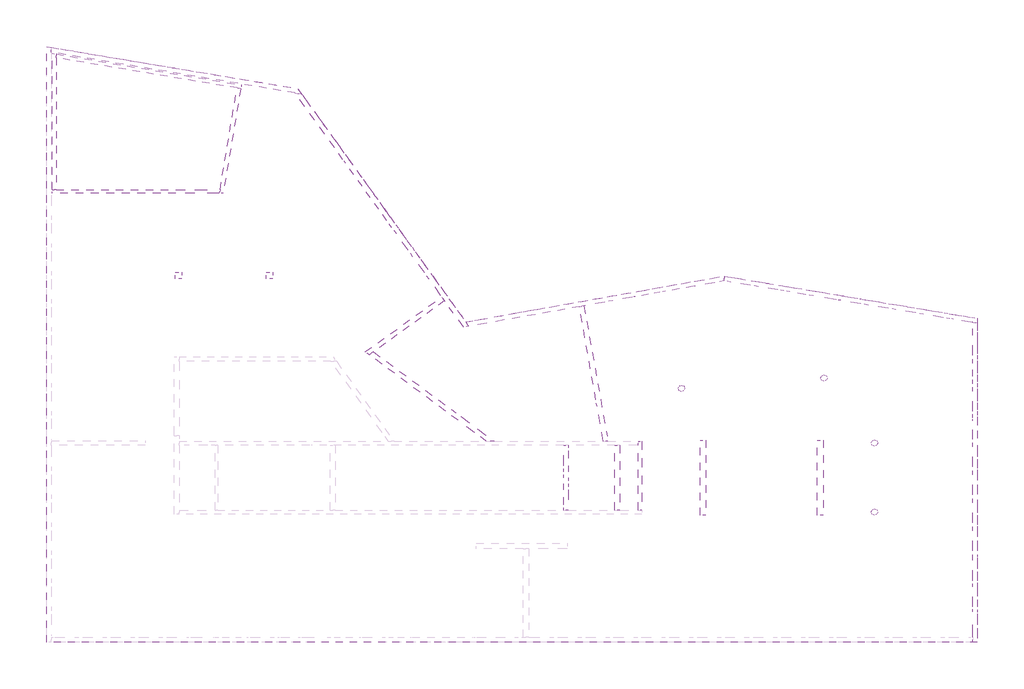
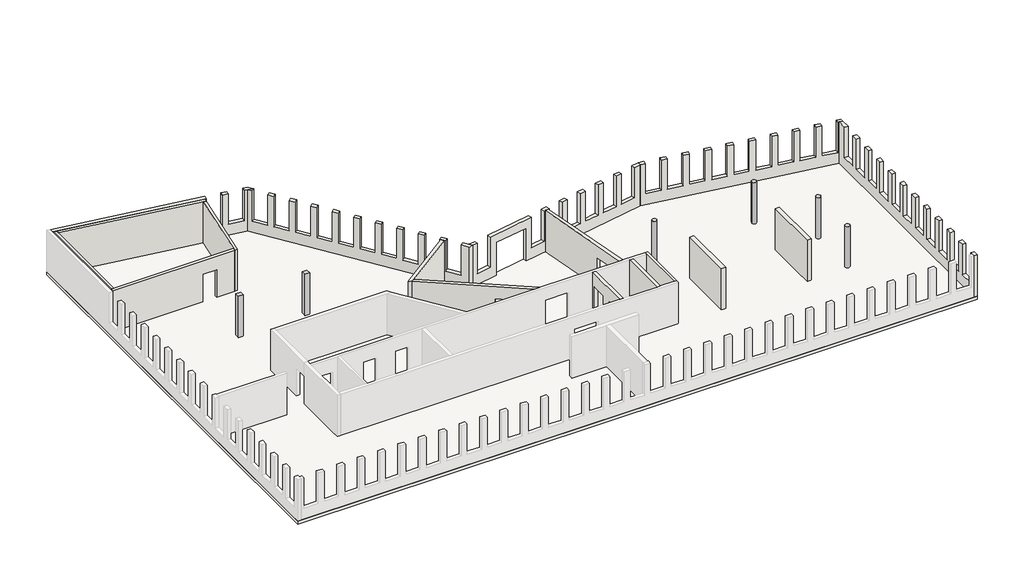
# One storey, part 2 of 2: 17 walls, 6 columns, 1 slab.
"""IFC4 building model written with IfcOpenShell, lengths in millimetres."""

from ifc_helpers import new_model, si_unit, point, frame, frame_2d, origin, place, context, project, spatial, polyline, circle_curve, trimmed, segment, composite_curve, outline, extrude, faceted_brep, element, save

model = new_model("IFC4")

# Units and contexts
model_context = context("Model", 3, world=origin())
ifc_project = project(units=[si_unit("LENGTHUNIT", "METRE", prefix="MILLI")], contexts=[model_context])

# Site, building, storey
site = spatial("IfcSite", under=ifc_project)
building = spatial("IfcBuilding", under=site)
storey = spatial("IfcBuildingStorey", under=building, Name="01_UG_OKFB_-4,20", Elevation=-4200.0)

# Columns
placement = place(None, origin())
element("IfcColumn", 1, ObjectType="5dki STB-Stützen rund : 5dki Stütze rund ø35cm C40/50", at=placement, inside=storey, context=model_context, shape_type="SweptSolid", body=[
    extrude(outline(composite_curve([segment(trimmed(circle_curve(frame_2d((33961.7583834, 13503.0230367)), 175.0), [point((34136.7583834, 13503.0230367))], [point((33786.7583834, 13503.0230367))], False, "CARTESIAN"), True, "CONTINUOUS"), segment(trimmed(circle_curve(frame_2d((33961.7583834, 13503.0230367)), 175.0), [point((33786.7583834, 13503.0230367))], [point((34136.7583834, 13503.0230367))], False, "CARTESIAN"), True, "CONTINUOUS")], self_intersect=False)), frame((0.0, 0.0, -150.0), z_axis=(0.0, 0.0, 1.0), x_axis=(1.0, 0.0, 0.0)), (0.0, 0.0, 1.0), 3210.0),
])
element("IfcColumn", 2, ObjectType="5dki STB-Stützen rechteckig : 5dki Stütze recht. 35x35cm C35/45", at=placement, inside=storey, context=model_context, shape_type="SweptSolid", body=[
    extrude(outline(polyline([(7139.9999521, 19742.0124565), (7139.9999521, 19392.0124565), (6789.9999521, 19392.0124565), (6789.9999521, 19742.0124565), (7139.9999521, 19742.0124565)])), frame((0.0, 0.0, -150.0), z_axis=(0.0, 0.0, 1.0), x_axis=(1.0, 0.0, 0.0)), (0.0, 0.0, 1.0), 3210.0),
])
element("IfcColumn", 3, ObjectType="5dki STB-Stützen rechteckig : 5dki Stütze recht. 35x35cm C35/45", at=placement, inside=storey, context=model_context, shape_type="SweptSolid", body=[
    extrude(outline(polyline([(12021.4450432, 19742.0124565), (12021.4450432, 19392.0124565), (11671.4450432, 19392.0124565), (11671.4450432, 19742.0124565), (12021.4450432, 19742.0124565)])), frame((0.0, 0.0, -150.0), z_axis=(0.0, 0.0, 1.0), x_axis=(1.0, 0.0, 0.0)), (0.0, 0.0, 1.0), 3210.0),
])
element("IfcColumn", 4, ObjectType="5dki STB-Stützen rund : 5dki Stütze rund ø35cm C40/50", at=placement, inside=storey, context=model_context, shape_type="SweptSolid", body=[
    extrude(outline(composite_curve([segment(trimmed(circle_curve(frame_2d((41616.0718251, 14052.9332427)), 175.0), [point((41791.0718251, 14052.9332427))], [point((41441.0718251, 14052.9332427))], False, "CARTESIAN"), True, "CONTINUOUS"), segment(trimmed(circle_curve(frame_2d((41616.0718251, 14052.9332427)), 175.0), [point((41441.0718251, 14052.9332427))], [point((41791.0718251, 14052.9332427))], False, "CARTESIAN"), True, "CONTINUOUS")], self_intersect=False)), frame((0.0, 0.0, -150.0), z_axis=(0.0, 0.0, 1.0), x_axis=(1.0, 0.0, 0.0)), (0.0, 0.0, 1.0), 3210.0),
])
element("IfcColumn", 5, ObjectType="5dki STB-Stützen rund : 5dki Stütze rund ø35cm C40/50", at=placement, inside=storey, context=model_context, shape_type="SweptSolid", body=[
    extrude(outline(composite_curve([segment(trimmed(circle_curve(frame_2d((44328.9990923, 10566.8309986)), 175.0), [point((44503.9990923, 10566.8309986))], [point((44153.9990923, 10566.8309986))], False, "CARTESIAN"), True, "CONTINUOUS"), segment(trimmed(circle_curve(frame_2d((44328.9990923, 10566.8309986)), 175.0), [point((44153.9990923, 10566.8309986))], [point((44503.9990923, 10566.8309986))], False, "CARTESIAN"), True, "CONTINUOUS")], self_intersect=False)), frame((0.0, 0.0, -150.0), z_axis=(0.0, 0.0, 1.0), x_axis=(1.0, 0.0, 0.0)), (0.0, 0.0, 1.0), 3210.0),
])
element("IfcColumn", 6, ObjectType="5dki STB-Stützen rund : 5dki Stütze rund ø35cm C40/50", at=placement, inside=storey, context=model_context, shape_type="SweptSolid", body=[
    extrude(outline(composite_curve([segment(trimmed(circle_curve(frame_2d((44328.9990923, 6852.1619165)), 175.0), [point((44503.9990923, 6852.1619165))], [point((44153.9990923, 6852.1619165))], False, "CARTESIAN"), True, "CONTINUOUS"), segment(trimmed(circle_curve(frame_2d((44328.9990923, 6852.1619165)), 175.0), [point((44153.9990923, 6852.1619165))], [point((44503.9990923, 6852.1619165))], False, "CARTESIAN"), True, "CONTINUOUS")], self_intersect=False)), frame((0.0, 0.0, -150.0), z_axis=(0.0, 0.0, 1.0), x_axis=(1.0, 0.0, 0.0)), (0.0, 0.0, 1.0), 3210.0),
])

# Slab
element("IfcSlab", 7, ObjectType="5dki Decke Ortbeton 25cm C30/37", at=placement, inside=storey, context=model_context, shape_type="SweptSolid", body=[
    extrude(outline(polyline([(13359.8955456, 29603.0548931), (22383.504194, 17069.412817), (36259.255712, 19532.4198889), (49863.9990834, 17260.5812626), (49863.9990834, -129.9989509), (-129.9989953, -129.9989509), (-129.9989953, 31855.7150729), (13359.8955456, 29603.0548931)]), holes=[polyline([(30391.9999833, 10442.0127412), (27891.9999829, 10442.0127412), (27891.9999829, 6960.0000515), (30391.9999833, 6960.0000515), (30391.9999833, 10442.0127412)]), polyline([(31652.9293554, 10442.0127466), (30641.9999891, 10442.0127466), (30641.9999891, 6948.5225137), (31652.9293554, 6948.5225137), (31652.9293554, 10442.0127466)]), polyline([(8916.9999838, 10442.0127045), (6990.0003593, 10442.0127045), (6990.0003593, 6960.0000208), (8916.9999838, 6960.0000208), (8916.9999838, 10442.0127045)]), polyline([(24127.0004657, 8820.0328918), (16927.0004692, 8820.0328918), (16927.0004692, 7020.033352), (24127.0004657, 7020.033352), (24127.0004657, 8820.0328918)])]), frame((0.0, 0.0, -400.0), z_axis=(0.0, 0.0, 1.0), x_axis=(1.0, 0.0, 0.0)), (0.0, 0.0, 1.0), 250.0),
])

# Walls
element("IfcWall", 8, ObjectType="5dki Lochfassade 26cm C30/37", at=placement, inside=storey, context=model_context, shape_type="Brep", body=[
    faceted_brep([(13575.6085618, 29303.4331075, 3060.0), (13211.4553837, 29364.2425792, 3060.0), (12991.7792945, 29400.9260074, 3060.0), (12991.7792945, 29400.9260074, 710.0), (11926.5295409, 29578.8106961, 710.0), (11926.5295409, 29578.8106961, 3060.0), (11512.2657479, 29647.9880751, 3060.0), (11512.2657479, 29647.9880751, 710.0), (10447.0159943, 29825.8727639, 710.0), (10447.0159943, 29825.8727639, 3060.0), (130.0010047, 31548.6978518, 3060.0), (130.0010047, 31548.6978518, -150.0), (13211.4553837, 29364.2425792, -150.0), (13575.6085618, 29303.4331075, -150.0), (13034.6033862, 29657.3750221, 710.0), (13034.6033862, 29657.3750221, 3060.0), (13359.8955383, 29603.0549033, 3060.0), (13359.8955383, 29603.0549033, -150.0), (130.0010047, 31812.2980067, -150.0), (130.0010047, 31812.2980067, 3060.0), (10489.840086, 30082.3217786, 3060.0), (10489.840086, 30082.3217786, 710.0), (11555.0898396, 29904.4370898, 710.0), (11555.0898396, 29904.4370898, 3060.0), (11969.3536327, 29835.2597109, 3060.0), (11969.3536327, 29835.2597109, 710.0)], [[[0, 1, 2, 3, 4, 5, 6, 7, 8, 9, 10, 11, 12, 13]], [[14, 15, 16, 17, 18, 19, 20, 21, 22, 23, 24, 25]], [[13, 12, 11, 18, 17]], [[19, 10, 9, 20]], [[24, 23, 6, 5]], [[16, 15, 2, 1, 0]], [[11, 10, 19, 18]], [[0, 13, 17, 16]], [[8, 21, 20, 9]], [[22, 7, 6, 23]], [[21, 8, 7, 22]], [[5, 4, 25, 24]], [[3, 2, 15, 14]], [[4, 3, 14, 25]]]),
])
element("IfcWall", 9, ObjectType="5dki Lochfassade 26cm C30/37", at=placement, inside=storey, context=model_context, shape_type="Brep", body=[
    faceted_brep([(22268.004401, 16784.8468851, 3060.0), (21924.4906268, 17261.9817942, 3060.0), (21924.4906268, 17261.9817942, 710.0), (21293.4697845, 18138.4592307, 710.0), (21293.4697845, 18138.4592307, 3060.0), (21048.0727903, 18479.3115671, 3060.0), (21048.0727903, 18479.3115671, 710.0), (20417.0519481, 19355.7890035, 710.0), (20417.0519481, 19355.7890035, 3060.0), (20171.6549538, 19696.64134, 3060.0), (20171.6549538, 19696.64134, 710.0), (19540.6341116, 20573.1187764, 710.0), (19540.6341116, 20573.1187764, 3060.0), (19295.2371174, 20913.9711128, 3060.0), (19295.2371174, 20913.9711128, 710.0), (18664.2162751, 21790.4485493, 710.0), (18664.2162751, 21790.4485493, 3060.0), (18418.8192809, 22131.3008857, 3060.0), (18418.8192809, 22131.3008857, 710.0), (17787.7984387, 23007.7783222, 710.0), (17787.7984387, 23007.7783222, 3060.0), (17542.4014445, 23348.6306586, 3060.0), (17542.4014445, 23348.6306586, 710.0), (16911.3806022, 24225.1080951, 710.0), (16911.3806022, 24225.1080951, 3060.0), (16665.983608, 24565.9604315, 3060.0), (16665.983608, 24565.9604315, 710.0), (16034.9627658, 25442.4378679, 710.0), (16034.9627658, 25442.4378679, 3060.0), (15789.5657715, 25783.2902043, 3060.0), (15789.5657715, 25783.2902043, 710.0), (15158.5449293, 26659.7676408, 710.0), (15158.5449293, 26659.7676408, 3060.0), (14913.1479351, 27000.6199772, 3060.0), (14913.1479351, 27000.6199772, 710.0), (14282.1270928, 27877.0974137, 710.0), (14282.1270928, 27877.0974137, 3060.0), (14036.7300986, 28217.9497501, 3060.0), (14036.7300986, 28217.9497501, 710.0), (13405.7092564, 29094.4271866, 710.0), (13405.7092564, 29094.4271866, 3060.0), (13211.4553837, 29364.2425792, 3060.0), (13211.4553837, 29364.2425792, -150.0), (22268.004401, 16784.8468851, -150.0), (22135.4944541, 17413.8942192, 710.0), (22135.4944541, 17413.8942192, 3060.0), (22383.5041721, 17069.4128529, 3060.0), (22552.0750732, 16835.2706799, 3060.0), (22552.0750732, 16835.2706799, -150.0), (22383.5041721, 17069.4128529, -150.0), (13575.6085618, 29303.4331075, -150.0), (13575.6085618, 29303.4331075, 3060.0), (13616.7130837, 29246.3396115, 3060.0), (13616.7130837, 29246.3396115, 710.0), (14247.7339259, 28369.8621751, 710.0), (14247.7339259, 28369.8621751, 3060.0), (14493.1309201, 28029.0098387, 3060.0), (14493.1309201, 28029.0098387, 710.0), (15124.1517624, 27152.5324022, 710.0), (15124.1517624, 27152.5324022, 3060.0), (15369.5487566, 26811.6800658, 3060.0), (15369.5487566, 26811.6800658, 710.0), (16000.5695988, 25935.2026293, 710.0), (16000.5695988, 25935.2026293, 3060.0), (16245.966593, 25594.3502929, 3060.0), (16245.966593, 25594.3502929, 710.0), (16876.9874353, 24717.8728564, 710.0), (16876.9874353, 24717.8728564, 3060.0), (17122.3844295, 24377.02052, 3060.0), (17122.3844295, 24377.02052, 710.0), (17753.4052718, 23500.5430836, 710.0), (17753.4052718, 23500.5430836, 3060.0), (17998.802266, 23159.6907472, 3060.0), (17998.802266, 23159.6907472, 710.0), (18629.8231082, 22283.2133107, 710.0), (18629.8231082, 22283.2133107, 3060.0), (18875.2201024, 21942.3609743, 3060.0), (18875.2201024, 21942.3609743, 710.0), (19506.2409447, 21065.8835378, 710.0), (19506.2409447, 21065.8835378, 3060.0), (19751.6379389, 20725.0312014, 3060.0), (19751.6379389, 20725.0312014, 710.0), (20382.6587811, 19848.5537649, 710.0), (20382.6587811, 19848.5537649, 3060.0), (20628.0557754, 19507.7014285, 3060.0), (20628.0557754, 19507.7014285, 710.0), (21259.0766176, 18631.2239921, 710.0), (21259.0766176, 18631.2239921, 3060.0), (21504.4736118, 18290.3716557, 3060.0), (21504.4736118, 18290.3716557, 710.0)], [[[0, 1, 2, 3, 4, 5, 6, 7, 8, 9, 10, 11, 12, 13, 14, 15, 16, 17, 18, 19, 20, 21, 22, 23, 24, 25, 26, 27, 28, 29, 30, 31, 32, 33, 34, 35, 36, 37, 38, 39, 40, 41, 42, 43]], [[44, 45, 46, 47, 48, 49, 50, 51, 52, 53, 54, 55, 56, 57, 58, 59, 60, 61, 62, 63, 64, 65, 66, 67, 68, 69, 70, 71, 72, 73, 74, 75, 76, 77, 78, 79, 80, 81, 82, 83, 84, 85, 86, 87, 88, 89]], [[43, 42, 50, 49, 48]], [[51, 41, 40, 52]], [[56, 55, 37, 36]], [[60, 59, 33, 32]], [[64, 63, 29, 28]], [[68, 67, 25, 24]], [[72, 71, 21, 20]], [[76, 75, 17, 16]], [[80, 79, 13, 12]], [[84, 83, 9, 8]], [[88, 87, 5, 4]], [[47, 46, 45, 1, 0]], [[42, 41, 51, 50]], [[0, 43, 48, 47]], [[39, 53, 52, 40]], [[54, 38, 37, 55]], [[53, 39, 38, 54]], [[36, 35, 57, 56]], [[34, 33, 59, 58]], [[35, 34, 58, 57]], [[32, 31, 61, 60]], [[30, 29, 63, 62]], [[31, 30, 62, 61]], [[28, 27, 65, 64]], [[26, 25, 67, 66]], [[27, 26, 66, 65]], [[24, 23, 69, 68]], [[22, 21, 71, 70]], [[23, 22, 70, 69]], [[20, 19, 73, 72]], [[18, 17, 75, 74]], [[19, 18, 74, 73]], [[16, 15, 77, 76]], [[14, 13, 79, 78]], [[15, 14, 78, 77]], [[12, 11, 81, 80]], [[10, 9, 83, 82]], [[11, 10, 82, 81]], [[8, 7, 85, 84]], [[6, 5, 87, 86]], [[7, 6, 86, 85]], [[4, 3, 89, 88]], [[2, 1, 45, 44]], [[3, 2, 44, 89]]]),
])
element("IfcWall", 10, ObjectType="5dki Lochfassade 26cm C30/37", at=placement, inside=storey, context=model_context, shape_type="Brep", body=[
    faceted_brep([(34703.2430153, 18992.1564787, 710.0), (34703.2430153, 18992.1564787, 3060.0), (34289.7072944, 18918.7520679, 3060.0), (34289.7072944, 18918.7520679, 710.0), (33226.3297263, 18729.9978686, 710.0), (33226.3297263, 18729.9978686, 3060.0), (32812.7940054, 18656.5934577, 3060.0), (32812.7940054, 18656.5934577, 710.0), (31749.4164374, 18467.8392585, 710.0), (31749.4164374, 18467.8392585, 3060.0), (31335.8807164, 18394.4348476, 3060.0), (31335.8807164, 18394.4348476, 710.0), (30272.5031484, 18205.6806483, 710.0), (30272.5031484, 18205.6806483, 3060.0), (29858.9674275, 18132.2762375, 3060.0), (29858.9674275, 18132.2762375, 710.0), (28795.5898594, 17943.5220382, 710.0), (28795.5898594, 17943.5220382, 3060.0), (28731.5904499, 17932.1618613, 3060.0), (28485.4382351, 17888.4687596, 3060.0), (28382.0541385, 17870.1176274, 3060.0), (28382.0541385, 17870.1176274, 710.0), (27318.6765704, 17681.3634281, 710.0), (27318.6765704, 17681.3634281, 3060.0), (23971.0064488, 17087.1372452, 3060.0), (23971.0064488, 17087.1372452, 710.0), (22907.6288807, 16898.3830459, 710.0), (22907.6288807, 16898.3830459, 3060.0), (22552.0750732, 16835.2706799, 3060.0), (22552.0750732, 16835.2706799, -150.0), (24463.3121553, 17174.5236752, -150.0), (24463.3121553, 17174.5236752, 2410.0), (26924.8343036, 17611.454692, 2410.0), (26924.8343036, 17611.454692, -150.0), (28485.4382351, 17888.4687596, -150.0), (28731.5904499, 17932.1618613, -150.0), (36261.33607, 19268.7248546, -150.0), (36261.33607, 19268.7248546, 3060.0), (35766.6205834, 19180.910678, 3060.0), (35766.6205834, 19180.910678, 710.0), (34244.2664686, 19174.7503713, 3060.0), (34657.8021895, 19248.1547821, 3060.0), (34657.8021895, 19248.1547821, 710.0), (35721.1797576, 19436.9089814, 710.0), (35721.1797576, 19436.9089814, 3060.0), (36259.9888873, 19532.5499737, 3060.0), (36259.9888873, 19532.5499737, -150.0), (26879.3934778, 17867.4529955, -150.0), (26879.3934778, 17867.4529955, 2410.0), (24417.8713295, 17430.5219786, 2410.0), (24417.8713295, 17430.5219786, -150.0), (22383.5041721, 17069.4128529, -150.0), (22383.5041721, 17069.4128529, 3060.0), (22862.188055, 17154.3813493, 3060.0), (22862.188055, 17154.3813493, 710.0), (23925.565623, 17343.1355486, 710.0), (23925.565623, 17343.1355486, 3060.0), (27273.2357447, 17937.3617315, 3060.0), (27273.2357447, 17937.3617315, 710.0), (28336.6133127, 18126.1159308, 710.0), (28336.6133127, 18126.1159308, 3060.0), (28750.1490337, 18199.5203416, 3060.0), (28750.1490337, 18199.5203416, 710.0), (29813.5266017, 18388.2745409, 710.0), (29813.5266017, 18388.2745409, 3060.0), (30227.0623226, 18461.6789518, 3060.0), (30227.0623226, 18461.6789518, 710.0), (31290.4398907, 18650.433151, 710.0), (31290.4398907, 18650.433151, 3060.0), (31703.9756116, 18723.8375619, 3060.0), (31703.9756116, 18723.8375619, 710.0), (32767.3531797, 18912.5917612, 710.0), (32767.3531797, 18912.5917612, 3060.0), (33180.8889006, 18985.996172, 3060.0), (33180.8889006, 18985.996172, 710.0), (34244.2664686, 19174.7503713, 710.0)], [[[0, 1, 2, 3, 4, 5, 6, 7, 8, 9, 10, 11, 12, 13, 14, 15, 16, 17, 18, 19, 20, 21, 22, 23, 24, 25, 26, 27, 28, 29, 30, 31, 32, 33, 34, 35, 36, 37, 38, 39]], [[40, 41, 42, 43, 44, 45, 46, 47, 48, 49, 50, 51, 52, 53, 54, 55, 56, 57, 58, 59, 60, 61, 62, 63, 64, 65, 66, 67, 68, 69, 70, 71, 72, 73, 74, 75]], [[29, 51, 50, 30]], [[46, 36, 35, 34, 33, 47]], [[53, 52, 28, 27]], [[24, 23, 57, 56]], [[61, 60, 20, 19, 18, 17]], [[14, 13, 65, 64]], [[69, 68, 10, 9]], [[6, 5, 73, 72]], [[38, 37, 45, 44]], [[2, 1, 41, 40]], [[29, 28, 52, 51]], [[37, 36, 46, 45]], [[49, 31, 30, 50]], [[31, 49, 48, 32]], [[32, 48, 47, 33]], [[27, 26, 54, 53]], [[25, 24, 56, 55]], [[26, 25, 55, 54]], [[60, 59, 21, 20]], [[58, 57, 23, 22]], [[59, 58, 22, 21]], [[17, 16, 62, 61]], [[15, 14, 64, 63]], [[16, 15, 63, 62]], [[68, 67, 11, 10]], [[66, 65, 13, 12]], [[67, 66, 12, 11]], [[9, 8, 70, 69]], [[7, 6, 72, 71]], [[8, 7, 71, 70]], [[40, 75, 3, 2]], [[74, 73, 5, 4]], [[75, 74, 4, 3]], [[44, 43, 39, 38]], [[42, 41, 1, 0]], [[43, 42, 0, 39]]]),
])
element("IfcWall", 11, ObjectType="5dki Lochfassade 26cm C30/37", at=placement, inside=storey, context=model_context, shape_type="Brep", body=[
    faceted_brep([(49863.9990837, 16997.2336245, 3060.0), (49603.9990837, 17040.6506907, 3060.0), (49507.8677901, 17056.7035319, 3060.0), (49507.8677901, 17056.7035319, 710.0), (48442.6180365, 17234.5882205, 710.0), (48442.6180365, 17234.5882205, 3060.0), (48028.3542434, 17303.7655993, 3060.0), (48028.3542434, 17303.7655993, 710.0), (46963.1044898, 17481.6502878, 710.0), (46963.1044898, 17481.6502878, 3060.0), (46548.8406967, 17550.8276667, 3060.0), (46548.8406967, 17550.8276667, 710.0), (45483.5909431, 17728.7123552, 710.0), (45483.5909431, 17728.7123552, 3060.0), (45069.32715, 17797.8897341, 3060.0), (45069.32715, 17797.8897341, 710.0), (44004.0773964, 17975.7744226, 710.0), (44004.0773964, 17975.7744226, 3060.0), (43589.8136033, 18044.9518015, 3060.0), (43589.8136033, 18044.9518015, 710.0), (42524.5638497, 18222.83649, 710.0), (42524.5638497, 18222.83649, 3060.0), (42110.3000566, 18292.0138689, 3060.0), (42110.3000566, 18292.0138689, 710.0), (41045.050303, 18469.8985574, 710.0), (41045.050303, 18469.8985574, 3060.0), (40630.7865099, 18539.0759362, 3060.0), (40630.7865099, 18539.0759362, 710.0), (39565.5367563, 18716.9606248, 710.0), (39565.5367563, 18716.9606248, 3060.0), (39151.2729632, 18786.1380036, 3060.0), (39151.2729632, 18786.1380036, 710.0), (38086.0232096, 18964.0226921, 710.0), (38086.0232096, 18964.0226921, 3060.0), (37671.7594165, 19033.200071, 3060.0), (37671.7594165, 19033.200071, 710.0), (36606.5096629, 19211.0847595, 710.0), (36606.5096629, 19211.0847595, 3060.0), (36261.33607, 19268.7248546, 3060.0), (36261.33607, 19268.7248546, -150.0), (49603.9990837, 17040.6506907, -150.0), (49863.9990837, 16997.2336245, -150.0), (49550.6918818, 17313.1525467, 710.0), (49550.6918818, 17313.1525467, 3060.0), (49863.9990833, 17260.8337794, 3060.0), (49863.9990833, 17260.8337794, -150.0), (36259.9888873, 19532.5499737, -150.0), (36259.9888873, 19532.5499737, 3060.0), (36649.3337546, 19467.5337743, 3060.0), (36649.3337546, 19467.5337743, 710.0), (37714.5835082, 19289.6490858, 710.0), (37714.5835082, 19289.6490858, 3060.0), (38128.8473013, 19220.4717069, 3060.0), (38128.8473013, 19220.4717069, 710.0), (39194.0970549, 19042.5870184, 710.0), (39194.0970549, 19042.5870184, 3060.0), (39608.360848, 18973.4096395, 3060.0), (39608.360848, 18973.4096395, 710.0), (40673.6106016, 18795.524951, 710.0), (40673.6106016, 18795.524951, 3060.0), (41087.8743947, 18726.3475721, 3060.0), (41087.8743947, 18726.3475721, 710.0), (42153.1241483, 18548.4628836, 710.0), (42153.1241483, 18548.4628836, 3060.0), (42567.3879414, 18479.2855048, 3060.0), (42567.3879414, 18479.2855048, 710.0), (43632.637695, 18301.4008162, 710.0), (43632.637695, 18301.4008162, 3060.0), (44046.9014881, 18232.2234374, 3060.0), (44046.9014881, 18232.2234374, 710.0), (45112.1512417, 18054.3387489, 710.0), (45112.1512417, 18054.3387489, 3060.0), (45526.4150348, 17985.16137, 3060.0), (45526.4150348, 17985.16137, 710.0), (46591.6647884, 17807.2766815, 710.0), (46591.6647884, 17807.2766815, 3060.0), (47005.9285815, 17738.0993026, 3060.0), (47005.9285815, 17738.0993026, 710.0), (48071.1783351, 17560.2146141, 710.0), (48071.1783351, 17560.2146141, 3060.0), (48485.4421282, 17491.0372352, 3060.0), (48485.4421282, 17491.0372352, 710.0)], [[[0, 1, 2, 3, 4, 5, 6, 7, 8, 9, 10, 11, 12, 13, 14, 15, 16, 17, 18, 19, 20, 21, 22, 23, 24, 25, 26, 27, 28, 29, 30, 31, 32, 33, 34, 35, 36, 37, 38, 39, 40, 41]], [[42, 43, 44, 45, 46, 47, 48, 49, 50, 51, 52, 53, 54, 55, 56, 57, 58, 59, 60, 61, 62, 63, 64, 65, 66, 67, 68, 69, 70, 71, 72, 73, 74, 75, 76, 77, 78, 79, 80, 81]], [[41, 40, 39, 46, 45]], [[48, 47, 38, 37]], [[52, 51, 34, 33]], [[56, 55, 30, 29]], [[60, 59, 26, 25]], [[64, 63, 22, 21]], [[68, 67, 18, 17]], [[72, 71, 14, 13]], [[76, 75, 10, 9]], [[80, 79, 6, 5]], [[44, 43, 2, 1, 0]], [[39, 38, 47, 46]], [[0, 41, 45, 44]], [[37, 36, 49, 48]], [[35, 34, 51, 50]], [[36, 35, 50, 49]], [[33, 32, 53, 52]], [[31, 30, 55, 54]], [[32, 31, 54, 53]], [[29, 28, 57, 56]], [[27, 26, 59, 58]], [[28, 27, 58, 57]], [[25, 24, 61, 60]], [[23, 22, 63, 62]], [[24, 23, 62, 61]], [[21, 20, 65, 64]], [[19, 18, 67, 66]], [[20, 19, 66, 65]], [[17, 16, 69, 68]], [[15, 14, 71, 70]], [[16, 15, 70, 69]], [[13, 12, 73, 72]], [[11, 10, 75, 74]], [[12, 11, 74, 73]], [[9, 8, 77, 76]], [[7, 6, 79, 78]], [[8, 7, 78, 77]], [[5, 4, 81, 80]], [[3, 2, 43, 42]], [[4, 3, 42, 81]]]),
])
element("IfcWall", 12, ObjectType="5dki Lochfassade 26cm C30/37", at=placement, inside=storey, context=model_context, shape_type="Brep", body=[
    faceted_brep([(49603.9991105, -129.9989514, 3060.0), (49603.9991101, 130.0010486, 3060.0), (49603.9991099, 277.0124979, 3060.0), (49603.9991099, 277.0124979, 710.0), (49603.9991082, 1357.0124979, 710.0), (49603.9991082, 1357.0124979, 3060.0), (49603.9991075, 1777.0124979, 3060.0), (49603.9991075, 1777.0124979, 710.0), (49603.9991058, 2857.0124979, 710.0), (49603.9991058, 2857.0124979, 3060.0), (49603.9991052, 3277.0124979, 3060.0), (49603.9991052, 3277.0124979, 710.0), (49603.9991035, 4357.0124979, 710.0), (49603.9991035, 4357.0124979, 3060.0), (49603.9991028, 4777.0124979, 3060.0), (49603.9991028, 4777.0124979, 710.0), (49603.9991011, 5857.0124979, 710.0), (49603.9991011, 5857.0124979, 3060.0), (49603.9991005, 6277.0124979, 3060.0), (49603.9991005, 6277.0124979, 710.0), (49603.9990988, 7357.0124979, 710.0), (49603.9990988, 7357.0124979, 3060.0), (49603.9990981, 7777.0124979, 3060.0), (49603.9990981, 7777.0124979, 710.0), (49603.9990964, 8857.0124979, 710.0), (49603.9990964, 8857.0124979, 3060.0), (49603.9990958, 9277.0124979, 3060.0), (49603.9990958, 9277.0124979, 710.0), (49603.9990941, 10357.0124979, 710.0), (49603.9990941, 10357.0124979, 3060.0), (49603.9990934, 10777.0124979, 3060.0), (49603.9990934, 10777.0124979, 710.0), (49603.9990918, 11857.0124979, 710.0), (49603.9990918, 11857.0124979, 3060.0), (49603.9990911, 12277.0124979, 3060.0), (49603.9990911, 12277.0124979, 710.0), (49603.9990894, 13357.0124979, 710.0), (49603.9990894, 13357.0124979, 3060.0), (49603.9990888, 13777.0124979, 3060.0), (49603.9990888, 13777.0124979, 710.0), (49603.9990871, 14857.0124979, 710.0), (49603.9990871, 14857.0124979, 3060.0), (49603.9990864, 15277.0124979, 3060.0), (49603.9990864, 15277.0124979, 710.0), (49603.9990847, 16357.0124979, 710.0), (49603.9990847, 16357.0124979, 3060.0), (49603.9990837, 17040.6506907, 3060.0), (49603.9990837, 17040.6506907, -150.0), (49603.9991101, 130.0010486, -150.0), (49603.9991105, -129.9989514, -150.0), (49863.9991099, 277.0124983, 710.0), (49863.9991099, 277.0124983, 3060.0), (49863.9991105, -129.9989509, 3060.0), (49863.9991105, -129.9989509, -150.0), (49863.9990837, 16997.2336245, -150.0), (49863.9990837, 16997.2336245, 3060.0), (49863.9990847, 16357.0124983, 3060.0), (49863.9990847, 16357.0124983, 710.0), (49863.9990864, 15277.0124983, 710.0), (49863.9990864, 15277.0124983, 3060.0), (49863.9990871, 14857.0124983, 3060.0), (49863.9990871, 14857.0124983, 710.0), (49863.9990888, 13777.0124983, 710.0), (49863.9990888, 13777.0124983, 3060.0), (49863.9990894, 13357.0124983, 3060.0), (49863.9990894, 13357.0124983, 710.0), (49863.9990911, 12277.0124983, 710.0), (49863.9990911, 12277.0124983, 3060.0), (49863.9990918, 11857.0124983, 3060.0), (49863.9990918, 11857.0124983, 710.0), (49863.9990934, 10777.0124983, 710.0), (49863.9990934, 10777.0124983, 3060.0), (49863.9990941, 10357.0124983, 3060.0), (49863.9990941, 10357.0124983, 710.0), (49863.9990958, 9277.0124983, 710.0), (49863.9990958, 9277.0124983, 3060.0), (49863.9990964, 8857.0124983, 3060.0), (49863.9990964, 8857.0124983, 710.0), (49863.9990981, 7777.0124983, 710.0), (49863.9990981, 7777.0124983, 3060.0), (49863.9990988, 7357.0124983, 3060.0), (49863.9990988, 7357.0124983, 710.0), (49863.9991005, 6277.0124983, 710.0), (49863.9991005, 6277.0124983, 3060.0), (49863.9991011, 5857.0124983, 3060.0), (49863.9991011, 5857.0124983, 710.0), (49863.9991028, 4777.0124983, 710.0), (49863.9991028, 4777.0124983, 3060.0), (49863.9991035, 4357.0124983, 3060.0), (49863.9991035, 4357.0124983, 710.0), (49863.9991052, 3277.0124983, 710.0), (49863.9991052, 3277.0124983, 3060.0), (49863.9991058, 2857.0124983, 3060.0), (49863.9991058, 2857.0124983, 710.0), (49863.9991075, 1777.0124983, 710.0), (49863.9991075, 1777.0124983, 3060.0), (49863.9991082, 1357.0124983, 3060.0), (49863.9991082, 1357.0124983, 710.0)], [[[0, 1, 2, 3, 4, 5, 6, 7, 8, 9, 10, 11, 12, 13, 14, 15, 16, 17, 18, 19, 20, 21, 22, 23, 24, 25, 26, 27, 28, 29, 30, 31, 32, 33, 34, 35, 36, 37, 38, 39, 40, 41, 42, 43, 44, 45, 46, 47, 48, 49]], [[50, 51, 52, 53, 54, 55, 56, 57, 58, 59, 60, 61, 62, 63, 64, 65, 66, 67, 68, 69, 70, 71, 72, 73, 74, 75, 76, 77, 78, 79, 80, 81, 82, 83, 84, 85, 86, 87, 88, 89, 90, 91, 92, 93, 94, 95, 96, 97]], [[49, 48, 47, 54, 53]], [[55, 46, 45, 56]], [[42, 41, 60, 59]], [[38, 37, 64, 63]], [[34, 33, 68, 67]], [[30, 29, 72, 71]], [[26, 25, 76, 75]], [[22, 21, 80, 79]], [[18, 17, 84, 83]], [[14, 13, 88, 87]], [[10, 9, 92, 91]], [[96, 95, 6, 5]], [[52, 51, 2, 1, 0]], [[47, 46, 55, 54]], [[0, 49, 53, 52]], [[58, 43, 42, 59]], [[44, 57, 56, 45]], [[43, 58, 57, 44]], [[63, 62, 39, 38]], [[61, 60, 41, 40]], [[62, 61, 40, 39]], [[67, 66, 35, 34]], [[65, 64, 37, 36]], [[66, 65, 36, 35]], [[71, 70, 31, 30]], [[69, 68, 33, 32]], [[70, 69, 32, 31]], [[75, 74, 27, 26]], [[73, 72, 29, 28]], [[74, 73, 28, 27]], [[79, 78, 23, 22]], [[77, 76, 25, 24]], [[78, 77, 24, 23]], [[83, 82, 19, 18]], [[81, 80, 21, 20]], [[82, 81, 20, 19]], [[87, 86, 15, 14]], [[85, 84, 17, 16]], [[86, 85, 16, 15]], [[91, 90, 11, 10]], [[89, 88, 13, 12]], [[90, 89, 12, 11]], [[95, 94, 7, 6]], [[93, 92, 9, 8]], [[94, 93, 8, 7]], [[5, 4, 97, 96]], [[3, 2, 51, 50]], [[4, 3, 50, 97]]]),
])
element("IfcWall", 13, ObjectType="5dki STB-Wand Kern 25cm C30/37", at=placement, inside=storey, context=model_context, shape_type="SweptSolid", body=[
    extrude(outline(polyline([(30641.9999891, 10442.0127483), (30641.9999891, 6960.0000501), (30391.9999891, 6960.0000498), (30391.9999891, 10442.0127479), (30641.9999891, 10442.0127483)])), frame((0.0, 0.0, -150.0), z_axis=(0.0, 0.0, 1.0), x_axis=(1.0, 0.0, 0.0)), (0.0, 0.0, 1.0), 3210.0),
])
element("IfcWall", 14, ObjectType="5dki STB-Wand Kern 25cm C30/37", at=placement, inside=storey, context=model_context, shape_type="SweptSolid", body=[
    extrude(outline(polyline([(3482.0126944, -3210.0), (-2.1e-06, -3210.0), (-2.1e-06, 0.0), (279.9681323, 0.0), (279.9681323, -2260.0), (1414.9681323, -2260.0), (1414.9681323, 0.0), (2067.1995869, 0.0), (2067.1995869, -2260.0), (3202.1995869, -2260.0), (3202.1995869, 0.0), (3482.0126944, 0.0), (3482.0126944, -3210.0)])), frame((27641.9999829, 10442.0127408, -150.0), z_axis=(1.0, 1.6300916066412081e-09, 0.0), x_axis=(1.6300916066412081e-09, -1.0, 0.0)), (0.0, 0.0, 1.0), 250.0),
])
element("IfcWall", 15, ObjectType="5dki STB-Wand Kern 20cm C35/45", at=placement, inside=storey, context=model_context, shape_type="Brep", body=[
    faceted_brep([(31641.9999912, 10662.0127502, -150.0), (31641.9999881, 10442.0127502, -150.0), (31641.9999382, 6960.0000514, -150.0), (31641.9999382, 6960.0000514, 3060.0), (31641.9999881, 10442.0127502, 3060.0), (31641.9999912, 10662.0127502, 3060.0), (31841.9999912, 10662.0127505, -150.0), (31841.9999912, 10662.0127505, 3060.0), (31841.9999382, 6960.0000516, 3060.0), (31841.9999382, 6960.0000516, -150.0)], [[[0, 1, 2, 3, 4, 5]], [[6, 7, 8, 9]], [[2, 1, 0, 6, 9]], [[5, 4, 3, 8, 7]], [[0, 5, 7, 6]], [[3, 2, 9, 8]]]),
])
element("IfcWall", 16, ObjectType="5dki STB-Wand 20cm C30/37", at=placement, inside=storey, context=model_context, shape_type="Brep", body=[
    faceted_brep([(179.9999842, 24166.8495132, 3060.0), (379.9999842, 24166.8495132, 3060.0), (9187.7304791, 24166.8495132, 3060.0), (9187.7304791, 24166.8495132, -150.0), (7830.000204, 24166.8495132, -150.0), (7830.000204, 24166.8495132, 1985.0), (6820.000204, 24166.8495132, 1985.0), (6820.000204, 24166.8495132, -150.0), (379.9999842, 24166.8495132, -150.0), (179.9999842, 24166.8495132, -150.0), (9154.332736, 23966.8495132, 3060.0), (179.9999842, 23966.8495132, 3060.0), (179.9999842, 23966.8495132, -150.0), (6820.000204, 23966.8495132, -150.0), (6820.000204, 23966.8495132, 1985.0), (7830.000204, 23966.8495132, 1985.0), (7830.000204, 23966.8495132, -150.0), (9154.332736, 23966.8495132, -150.0)], [[[0, 1, 2, 3, 4, 5, 6, 7, 8, 9]], [[10, 11, 12, 13, 14, 15, 16, 17]], [[12, 9, 8, 7, 13]], [[3, 17, 16, 4]], [[2, 1, 0, 11, 10]], [[0, 9, 12, 11]], [[3, 2, 10, 17]], [[15, 5, 4, 16]], [[5, 15, 14, 6]], [[6, 14, 13, 7]]]),
])
element("IfcWall", 17, ObjectType="5dki STB-Wand 20cm C30/37", at=placement, inside=storey, context=model_context, shape_type="Brep", body=[
    faceted_brep([(379.9999842, 24166.8495132, -150.0), (379.9999842, 31253.489127, -150.0), (379.9999842, 31456.2584769, -150.0), (379.9999842, 31456.2584769, 3060.0), (379.9999842, 31253.489127, 3060.0), (379.9999842, 24166.8495132, 3060.0), (179.9999842, 24166.8495132, -150.0), (179.9999842, 24166.8495132, 3060.0), (179.9999842, 31489.6562201, 3060.0), (179.9999842, 31489.6562201, -150.0)], [[[0, 1, 2, 3, 4, 5]], [[6, 7, 8, 9]], [[2, 1, 0, 6, 9]], [[5, 4, 3, 8, 7]], [[0, 5, 7, 6]], [[3, 2, 9, 8]]]),
])
element("IfcWall", 18, ObjectType="5dki STB-Wand 20cm C30/37", at=placement, inside=storey, context=model_context, shape_type="Brep", body=[
    faceted_brep([(379.9999842, 31253.489127, -150.0), (10100.0728462, 29630.3466386, -150.0), (10297.3413191, 29597.4050296, -150.0), (10297.3413191, 29597.4050296, 3060.0), (10100.0728462, 29630.3466386, 3060.0), (379.9999842, 31253.489127, 3060.0), (379.9999842, 31456.2584769, -150.0), (379.9999842, 31456.2584769, 3060.0), (10330.282928, 29794.6735025, 3060.0), (10330.282928, 29794.6735025, -150.0)], [[[0, 1, 2, 3, 4, 5]], [[6, 7, 8, 9]], [[2, 1, 0, 6, 9]], [[5, 4, 3, 8, 7]], [[0, 5, 7, 6]], [[3, 2, 9, 8]]]),
])
element("IfcWall", 19, ObjectType="5dki STB-Wand 20cm C30/37", at=placement, inside=storey, context=model_context, shape_type="Brep", body=[
    faceted_brep([(10100.0728462, 29630.3466386, -150.0), (9187.7304791, 24166.8495132, -150.0), (9154.332736, 23966.8495132, -150.0), (9154.332736, 23966.8495132, 3060.0), (9187.7304791, 24166.8495132, 3060.0), (10100.0728462, 29630.3466386, 3060.0), (10297.3413191, 29597.4050296, -150.0), (10297.3413191, 29597.4050296, 3060.0), (9357.1020859, 23966.8495132, 3060.0), (9357.1020859, 23966.8495132, -150.0)], [[[0, 1, 2, 3, 4, 5]], [[6, 7, 8, 9]], [[2, 1, 0, 6, 9]], [[5, 4, 3, 8, 7]], [[0, 5, 7, 6]], [[3, 2, 9, 8]]]),
])
element("IfcWall", 20, ObjectType="5dki STB-Wand 25cm C30/37", at=placement, inside=storey, context=model_context, shape_type="Brep", body=[
    faceted_brep([(21084.845921, 18397.4352698, -150.0), (16996.4717259, 15463.7807738, -150.0), (16996.4717259, 15463.7807738, 3060.0), (21084.845921, 18397.4352698, 3060.0), (21230.5955347, 18194.3169542, -150.0), (21230.5955347, 18194.3169542, 3060.0), (17421.0951098, 15460.7711691, 3060.0), (17207.6873918, 15307.63829, 3060.0), (17207.6873918, 15307.63829, -150.0), (17421.0951098, 15460.7711691, -150.0)], [[[0, 1, 2, 3]], [[4, 5, 6, 7, 8, 9]], [[1, 0, 4, 9, 8]], [[3, 2, 7, 6, 5]], [[0, 3, 5, 4]], [[2, 1, 8, 7]]]),
])
element("IfcWall", 21, ObjectType="5dki STB-Wand 25cm C30/37", at=placement, inside=storey, context=model_context, shape_type="Brep", body=[
    faceted_brep([(23491.8764947, 10662.0127353, 3060.0), (17207.6873918, 15307.63829, 3060.0), (17207.6873918, 15307.63829, -150.0), (21455.778452, 12167.2107719, -150.0), (21455.778452, 12167.2107719, 2110.0), (22871.0433991, 11120.9674304, 2110.0), (22871.0433991, 11120.9674304, -150.0), (23491.8764947, 10662.0127353, -150.0), (17421.0951098, 15460.7711691, 3060.0), (23912.428752, 10662.0127361, 3060.0), (23912.428752, 10662.0127361, -150.0), (23019.6575101, 11321.9993832, -150.0), (23019.6575101, 11321.9993832, 2110.0), (21604.392563, 12368.2427246, 2110.0), (21604.392563, 12368.2427246, -150.0), (17421.0951098, 15460.7711691, -150.0)], [[[0, 1, 2, 3, 4, 5, 6, 7]], [[8, 9, 10, 11, 12, 13, 14, 15]], [[2, 15, 14, 3]], [[10, 7, 6, 11]], [[1, 0, 9, 8]], [[2, 1, 8, 15]], [[0, 7, 10, 9]], [[5, 12, 11, 6]], [[12, 5, 4, 13]], [[13, 4, 3, 14]]]),
])
element("IfcWall", 22, ObjectType="5dki STB-Wand 25cm C30/37", at=placement, inside=storey, context=model_context, shape_type="Brep", body=[
    faceted_brep([(29768.165987, 10662.0127467, 3060.0), (28485.4382351, 17888.4687596, 3060.0), (28485.4382351, 17888.4687596, -150.0), (29375.0297859, 12876.809659, -150.0), (29375.0297859, 12876.809659, 2110.0), (29682.6292216, 11143.8980666, 2110.0), (29682.6292216, 11143.8980666, -150.0), (29768.165987, 10662.0127467, -150.0), (28731.5904499, 17932.1618613, 3060.0), (30022.0739196, 10662.0127472, 3060.0), (30022.0739196, 10662.0127472, -150.0), (29928.7814364, 11187.5911682, -150.0), (29928.7814364, 11187.5911682, 2110.0), (29621.1820008, 12920.5027606, 2110.0), (29621.1820008, 12920.5027606, -150.0), (28731.5904499, 17932.1618613, -150.0)], [[[0, 1, 2, 3, 4, 5, 6, 7]], [[8, 9, 10, 11, 12, 13, 14, 15]], [[2, 15, 14, 3]], [[10, 7, 6, 11]], [[1, 0, 9, 8]], [[2, 1, 8, 15]], [[0, 7, 10, 9]], [[5, 12, 11, 6]], [[12, 5, 4, 13]], [[13, 4, 3, 14]]]),
])
element("IfcWall", 23, ObjectType="5dki STB-Wand 30cm C30/37", at=placement, inside=storey, context=model_context, shape_type="SweptSolid", body=[
    extrude(outline(polyline([(34969.9990839, 6680.0000532), (34969.9990776, 10702.0125181), (35269.9990776, 10702.0125186), (35269.9990839, 6680.0000537), (34969.9990839, 6680.0000532)])), frame((0.0, 0.0, -150.0), z_axis=(0.0, 0.0, 1.0), x_axis=(1.0, 0.0, 0.0)), (0.0, 0.0, 1.0), 3210.0),
])
element("IfcWall", 24, ObjectType="5dki STB-Wand 30cm C30/37", at=placement, inside=storey, context=model_context, shape_type="SweptSolid", body=[
    extrude(outline(polyline([(41269.9990703, 6680.000074), (41269.9990703, 10722.0122605), (41569.9990703, 10722.0122605), (41569.9990703, 6680.000074), (41269.9990703, 6680.000074)])), frame((0.0, 0.0, -150.0), z_axis=(0.0, 0.0, 1.0), x_axis=(1.0, 0.0, 0.0)), (0.0, 0.0, 1.0), 3210.0),
])

save(model, "model.ifc")

# Revit data of these elements
# Type "5dki STB-Stützen rund : 5dki Stütze rund ø35cm C40/50"
#   cpiFitMatchKey = "5D-KI-STB-OB-ST-RUN"
#   cpiComponentType = "Column"
#   5d Materialgüte = "C40/50"
#   Radius = 0.175 m
#   Durchmesser = 0.350 m
#   5dki Bewehrung Stab kg pro m3 = 0
#   5dki Sichtbeton SB3/SB4 [instance default] = no
#   Structural Material = 5d Beton - Stahlbeton
#   Assembly Code = ""
# Type "5dki STB-Stützen rechteckig : 5dki Stütze recht. 35x35cm C35/45"
#   cpiFitMatchKey = "5D-KI-STB-OB-ST-REC"
#   cpiComponentType = "Column"
#   5d Materialgüte = "C35/45"
#   Tiefe = 0.350 m
#   Breite = 0.350 m
#   5dki Bewehrung Stab kg pro m3 = 0
#   5dki Sichtbeton SB3/SB4 [instance default] = no
#   Structural Material = 5d Beton - Stahlbeton
#   Assembly Code = ""
# Type "5dki Decke Ortbeton 25cm C30/37"
#   cpiComponentType = "Slab"
#   cpiFitMatchKey = "5D-KI-STB-OB-DE"
#   5d Materialgüte = "C30/37"
#   Function = 0
#   5dki WU = no
#   Layers, outside or top first: 0.250 m "5d Beton - Stahlbeton" (function 1)
# Type "5dki Lochfassade 26cm C30/37"
#   Type Comments = ""
#   Description = ""
#   cpiComponentType = "Wall"
#   cpiFitMatchKey = "5D-KI-STB-OB-W-LF"
#   5d Materialgüte = "C35/45"
#   Filter Tragend / Nichttragend = yes
#   5dki WU = no
#   Layers, outside or top first: 0.260 m "5d Beton - Stahlbeton" (function 1)
# Type "5dki STB-Wand Kern 25cm C30/37"
#   Type Comments = ""
#   Description = ""
#   cpiComponentType = "Wall"
#   cpiFitMatchKey = "5D-KI-STB-OB-W-K"
#   5d Materialgüte = "C30/37"
#   Filter Tragend / Nichttragend = yes
#   5dki WU = no
#   Layers, outside or top first: 0.250 m "5d Beton - Stahlbeton" (function 1)
# Type "5dki STB-Wand Kern 20cm C35/45"
#   Type Comments = ""
#   Description = ""
#   cpiComponentType = "Wall"
#   cpiFitMatchKey = "5D-KI-STB-OB-W-K"
#   5d Materialgüte = "C35/45"
#   Filter Tragend / Nichttragend = yes
#   5dki WU = no
#   Layers, outside or top first: 0.200 m "5d Beton - Stahlbeton" (function 1)
# Type "5dki STB-Wand 20cm C30/37"
#   Type Comments = ""
#   Description = ""
#   cpiComponentType = "Wall"
#   cpiFitMatchKey = "5D-KI-STB-OB-W"
#   5d Materialgüte = "C30/37"
#   Filter Tragend / Nichttragend = yes
#   5dki WU = no
#   Layers, outside or top first: 0.200 m "5d Beton - Stahlbeton" (function 1)
# Type "5dki STB-Wand 25cm C30/37"
#   Type Comments = ""
#   Description = ""
#   cpiComponentType = "Wall"
#   cpiFitMatchKey = "5D-KI-STB-OB-W"
#   5d Materialgüte = "C30/37"
#   Filter Tragend / Nichttragend = yes
#   5dki WU = no
#   Layers, outside or top first: 0.250 m "5d Beton - Stahlbeton" (function 1)
# Type "5dki STB-Wand 30cm C30/37"
#   Type Comments = ""
#   Description = ""
#   cpiComponentType = "Wall"
#   cpiFitMatchKey = "5D-KI-STB-OB-W"
#   5d Materialgüte = "C30/37"
#   Filter Tragend / Nichttragend = yes
#   5dki WU = no
#   Layers, outside or top first: 0.300 m "5d Beton - Stahlbeton" (function 1)
# Element 1 (IfcColumn, "5dki STB-Stützen rund : 5dki Stütze rund ø35cm C40/50")
#   Comments = ""
#   000_080_030_Geschoß = "00_EG"
#   5dki Sichtbeton SB3/SB4 = no
#   Phase Created = Neu
#   Materials on its faces: "5d Beton - Stahlbeton"
# Element 2 (IfcColumn, "5dki STB-Stützen rechteckig : 5dki Stütze recht. 35x35cm C35/45")
#   Comments = ""
#   000_080_030_Geschoß = "00_EG"
#   5dki Sichtbeton SB3/SB4 = no
#   Phase Created = Neu
#   Materials on its faces: "5d Beton - Stahlbeton"
# Element 3 (IfcColumn, "5dki STB-Stützen rechteckig : 5dki Stütze recht. 35x35cm C35/45")
#   000_080_030_Geschoß = "00_EG"
#   5dki Sichtbeton SB3/SB4 = no
#   Phase Created = Neu
#   Materials on its faces: "5d Beton - Stahlbeton"
# Elements 4, 5, 6 (IfcColumn, "5dki STB-Stützen rund : 5dki Stütze rund ø35cm C40/50")
#   000_080_030_Geschoß = "00_EG"
#   5dki Sichtbeton SB3/SB4 = no
#   Phase Created = Neu
#   Materials on its faces: "5d Beton - Stahlbeton"
# Element 7 (IfcSlab, "5dki Decke Ortbeton 25cm C30/37")
#   000_080_030_Geschoß = "01_UG"
#   built-in parameter 1001955 = -0.165462 (stored number, unit not read)
#   Height Offset From Level = 0.000 m
#   built-in parameter 1001954 = 1
#   Phase Created = Neu
#   Materials on its faces: "5d Beton - Stahlbeton"
# Elements 8, 9, 10, 11, 12 (IfcWall, "5dki Lochfassade 26cm C30/37")
#   Comments = ""
#   000_080_030_Geschoß = "00_EG"
#   Top Offset = 0.000 m
#   Base Offset = 0.000 m
#   wall height = 3.210 m
#   Phase Created = Neu
#   Base Constraint = 01_UG_OKRD_-0,15
#   Top Constraint = 00_EG_UKRD_3,06
#   Materials on its faces: "5d Beton - Stahlbeton"
# Elements 13, 14 (IfcWall, "5dki STB-Wand Kern 25cm C30/37")
#   Comments = ""
#   000_080_030_Geschoß = "00_EG"
#   Top Offset = 0.000 m
#   Base Offset = 0.000 m
#   wall height = 3.210 m
#   Phase Created = Neu
#   Base Constraint = 01_UG_OKRD_-0,15
#   Top Constraint = 00_EG_UKRD_3,06
#   Materials on its faces: "5d Beton - Stahlbeton"
# Element 15 (IfcWall, "5dki STB-Wand Kern 20cm C35/45")
#   Comments = ""
#   000_080_030_Geschoß = "00_EG"
#   Top Offset = 0.000 m
#   Base Offset = 0.000 m
#   wall height = 3.210 m
#   Phase Created = Neu
#   Base Constraint = 01_UG_OKRD_-0,15
#   Top Constraint = 00_EG_UKRD_3,06
#   Materials on its faces: "5d Beton - Stahlbeton"
# Elements 16, 17, 18, 19 (IfcWall, "5dki STB-Wand 20cm C30/37")
#   Comments = ""
#   000_080_030_Geschoß = "00_EG"
#   Top Offset = 0.000 m
#   Base Offset = 0.000 m
#   wall height = 3.210 m
#   Phase Created = Neu
#   Base Constraint = 01_UG_OKRD_-0,15
#   Top Constraint = 00_EG_UKRD_3,06
#   Materials on its faces: "5d Beton - Stahlbeton"
# Elements 20, 21, 22 (IfcWall, "5dki STB-Wand 25cm C30/37")
#   Comments = ""
#   000_080_030_Geschoß = "00_EG"
#   Top Offset = 0.000 m
#   Base Offset = 0.000 m
#   wall height = 3.210 m
#   Phase Created = Neu
#   Base Constraint = 01_UG_OKRD_-0,15
#   Top Constraint = 00_EG_UKRD_3,06
#   Materials on its faces: "5d Beton - Stahlbeton"
# Element 23 (IfcWall, "5dki STB-Wand 30cm C30/37")
#   000_080_030_Geschoß = "00_EG"
#   Top Offset = 0.000 m
#   Base Offset = 0.000 m
#   wall height = 3.210 m
#   Phase Created = Neu
#   Base Constraint = 01_UG_OKRD_-0,15
#   Top Constraint = 00_EG_UKRD_3,06
#   Materials on its faces: "5d Beton - Stahlbeton"
# Element 24 (IfcWall, "5dki STB-Wand 30cm C30/37")
#   Comments = ""
#   000_080_030_Geschoß = "00_EG"
#   Top Offset = 0.000 m
#   Base Offset = 0.000 m
#   wall height = 3.210 m
#   Phase Created = Neu
#   Base Constraint = 01_UG_OKRD_-0,15
#   Top Constraint = 00_EG_UKRD_3,06
#   Materials on its faces: "5d Beton - Stahlbeton"
# Materials
#   "5d Beton - Stahlbeton": class "5dki", colour RGB 200 200 200, transparency 0, Cost = 0
